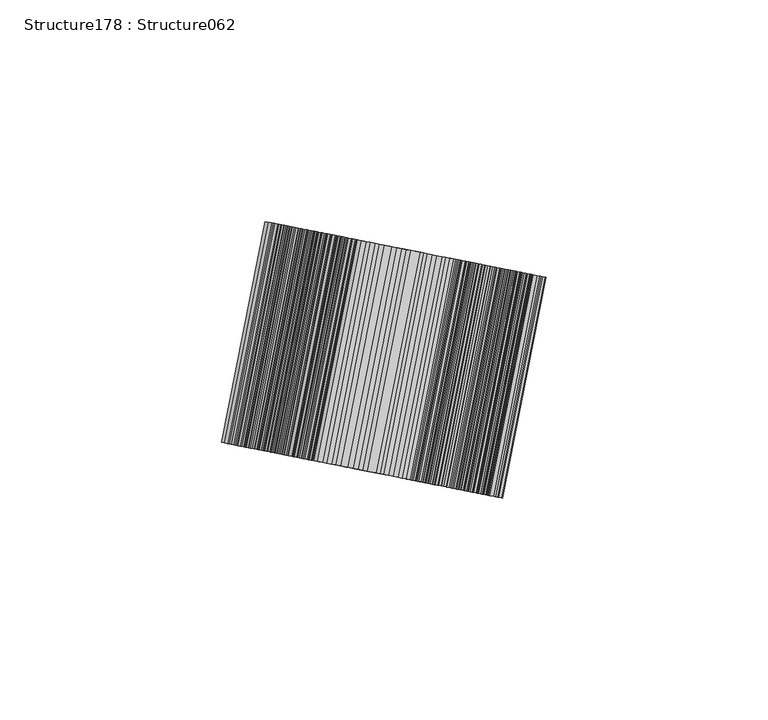
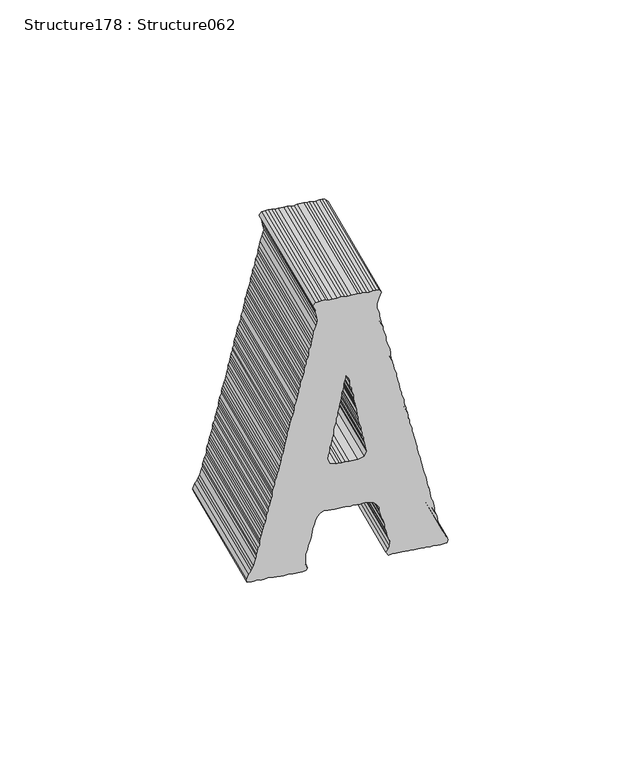
"""IFC4 building model written with IfcOpenShell, lengths in millimetres: proxy geometry, Structure178 : Structure062."""

from ifc_helpers import new_model, si_unit, frame, origin, place, context, project, spatial, polyline, outline, extrude, source, transform, mapped, element, save


def structure178_structure062_75744fdd(model_context):
    return source(origin(), model_context, "Body", "SweptSolid", [
        extrude(outline(polyline([(0.9094651, 0.0), (2.0811665, -0.5191353), (2.9906316, -0.6475848), (4.1562841, -0.7760343), (5.1991801, -1.1663642), (5.9748585, -1.299795), (7.1504738, -1.6851435), (8.1894559, -1.6851435), (9.3551084, -2.0758292), (10.2645735, -2.3377097), (11.4362748, -2.5946087), (12.3453841, -2.8564891), (13.3818755, -2.9849386), (14.1582655, -3.3752685), (15.4626861, -3.5040738), (16.3721513, -3.5040738), (17.5385154, -3.7659542), (19.491944, -4.4181645), (20.2718921, -4.6750635), (21.3101626, -4.9369439), (22.3470097, -4.9369439), (23.2561191, -5.1941987), (24.4278204, -5.5845287), (25.4700048, -5.9748585), (26.6363689, -5.9748585), (27.4124031, -6.3651884), (28.7175354, -6.6220874), (30.535754, -7.0127732), (31.5743802, -7.1462041), (32.7400327, -7.4031031), (33.6555467, -7.7934329), (35.4741211, -7.7934329), (36.5102567, -7.5315526), (37.5492387, -7.2746536), (38.3288311, -6.8843237), (39.3671015, -6.3651884), (40.4099976, -7.2746536), (40.5395145, -8.1837628), (40.5395145, -9.093228), (40.2826155, -10.2645735), (40.2826155, -11.3021323), (40.5395145, -12.4684964), (40.4099976, -13.2491562), (40.5395145, -14.1586213), (40.5395145, -16.2390762), (40.2826155, -17.2769908), (40.2826155, -18.3195311), (40.5395145, -19.4858951), (40.4099976, -20.6572406), (40.4099976, -22.3423842), (40.2826155, -23.5137297), (40.5395145, -24.422839), (40.5395145, -25.5941845), (40.4099976, -26.5032939), (40.2826155, -27.6746394), (39.2382962, -28.4506736), (38.3288311, -27.9315384), (37.4197218, -27.6746394), (36.6397736, -27.5412084), (35.4741211, -27.2843094), (33.5199809, -26.8939796), (32.6112274, -27.1508785), (31.4448633, -27.4127589), (29.3636968, -28.1934188), (27.545834, -28.4506736), (26.5089869, -28.712554), (25.3372855, -28.8410035), (24.2943895, -29.102884), (23.2561191, -29.6216633), (21.3101626, -29.7501128), (20.2718921, -30.012349), (19.491944, -30.5311284), (18.3202426, -30.5311284), (17.2816164, -30.9214584), (16.3721513, -31.1833388), (15.3356599, -31.1833388), (14.1582655, -31.4402377), (13.1253323, -31.8309234), (12.2158672, -32.2212534), (11.4362748, -32.3497029), (10.2645735, -32.4781524), (9.3551083, -32.8684823), (8.1894559, -32.8684823), (7.1504738, -33.259168), (6.2374505, -33.3876175), (5.0714422, -33.6494978), (3.2475306, -34.2967268), (2.0811665, -34.2967268), (1.1720572, -34.5586072), (0.1334309, -34.815862), (-1.0382704, -35.3396229), (-1.8178628, -35.4680724), (-2.8568449, -35.7249713), (-3.8990293, -35.8584022), (-5.0653934, -36.2487321), (-5.8471206, -36.5059869), (-7.0166871, -36.5059869), (-8.1826954, -36.8963168), (-8.9644226, -37.0297478), (-10.1364798, -37.4150963), (-11.1690572, -37.5485272), (-12.2115974, -37.6769766), (-12.9915456, -37.938857), (-14.03373, -38.3245613), (-15.3292552, -38.4579923), (-16.3678815, -38.7148912), (-18.1861001, -39.1052212), (-19.3581573, -39.3671016), (-20.2672666, -39.7528059), (-21.4371888, -40.0146862), (-22.2189161, -40.2765667), (-23.1223323, -40.5334657), (-24.1648726, -40.5334657), (-25.465735, -41.0572265), (-26.5025822, -41.3141255), (-27.4173846, -41.4429308), (-28.4560108, -41.4429308), (-29.235959, -41.7048112), (-30.5311284, -42.0951412), (-31.3110766, -42.2235906), (-32.3536168, -42.6139205), (-33.5214042, -42.6139205), (-34.4308693, -43.1330557), (-35.3399786, -43.3949362), (-36.37647, -43.3949362), (-37.5424783, -43.6568166), (-38.7202285, -44.0421651), (-39.6236447, -44.3040454), (-40.405372, -44.5659258), (-41.5752942, -44.6897497), (-42.6139205, -45.0850611), (-43.7856218, -45.3419601), (-44.8221132, -45.3419601), (-45.7372714, -45.4704096), (-46.6406876, -45.9941704), (-47.812389, -46.2510694), (-48.8510152, -46.5133056), (-49.7601245, -46.5133056), (-50.6731478, -46.9036355), (-52.8777823, -47.5508644), (-53.7929405, -47.9411943), (-54.5689747, -48.3318801), (-55.738897, -49.1125398), (-57.5532016, -49.7601246), (-58.4665807, -49.5028697), (-58.5957419, -48.1984491), (-58.4665807, -47.4224149), (-58.3331498, -46.2510694), (-58.5957419, -45.2135106), (-58.5957419, -44.0421651), (-58.3331498, -43.0042504), (-58.3331498, -42.0951412), (-58.4665807, -41.0572265), (-58.4665807, -40.1481172), (-58.5957419, -38.8433407), (-58.5957419, -37.938857), (-58.4665807, -36.8963168), (-58.3331498, -35.7249713), (-58.5957419, -34.815862), (-58.5957419, -31.8309234), (-58.3331498, -30.6595779), (-57.4297336, -30.1407985), (-56.6480063, -30.5311284), (-55.6115149, -30.7880274), (-53.3972734, -30.7880274), (-52.3586471, -30.7880274), (-51.4495378, -30.5311284), (-50.6731478, -30.1407985), (-49.3683714, -30.012349), (-48.4592621, -29.7501128), (-47.5497969, -29.3597829), (-46.6406876, -29.102884), (-45.6038405, -28.8410035), (-43.2661308, -28.5841045), (-41.5752942, -27.9315384), (-40.2762109, -27.6746394), (-38.9767716, -27.022429), (-38.1950444, -26.112964), (-37.4190102, -24.6847195), (-37.6759092, -23.6471606), (-37.6759092, -21.56635), (-37.5424783, -20.2669108), (-37.5424783, -17.5388712), (-37.6759092, -16.3675257), (-37.4190102, -15.4584164), (-37.5424783, -14.4205017), (-37.6759092, -13.3825872), (-37.5424783, -12.4684964), (-37.4190102, -11.1736828), (-37.6759092, -10.393023), (-38.0676623, -8.836329), (-38.8476105, -8.0503319), (-40.2762109, -7.0127732), (-41.4422191, -7.0127732), (-42.6139205, -6.7555183), (-44.561656, -6.2367389), (-45.3472973, -5.7129781), (-46.5133056, -5.4560792), (-47.2932538, -5.3276297), (-48.33188, -5.3276297), (-49.3683714, -4.803513), (-50.4126907, -4.6750635), (-51.4495378, -4.546614), (-52.3586471, -4.1562841), (-53.6595096, -3.7659542), (-55.3489229, -3.8944037), (-56.6480063, -4.2847336), (-57.2966585, -4.9369439), (-58.5957419, -4.1562841), (-58.4665807, -2.9849386), (-58.3331498, -1.9473797), (-58.3331498, 0.1334309), (-58.4665807, 1.1709896), (-58.4665807, 2.2089043), (-58.3331498, 3.1183694), (-58.4665807, 4.0274787), (-58.4665807, 5.3272737), (-58.3331498, 6.1079336), (-58.4665807, 7.4077285), (-58.3331498, 8.1887442), (-58.5957419, 9.2263031), (-58.3331498, 10.3976485), (-58.5957419, 11.5640127), (-58.4665807, 12.473122), (-58.3331498, 13.516018), (-58.3331498, 14.5535768), (-57.2966585, 14.9442625), (-56.3875492, 14.6823821), (-55.738897, 14.0347974), (-54.5689747, 13.7729169), (-53.7929405, 13.3825871), (-52.6151903, 12.8634519), (-50.6731478, 11.9543425), (-49.8875066, 11.6974435), (-48.5941162, 11.5640127), (-47.5497969, 11.3067579), (-46.6406876, 11.0448775), (-45.8646534, 10.6545475), (-44.561656, 10.526098), (-42.6139205, 10.2642176), (-41.4422191, 9.8788691), (-40.5384471, 9.4832021), (-39.6236447, 9.2263031), (-38.4576364, 9.0978536), (-37.4190102, 8.9644226), (-36.5059869, 8.8359731), (-35.6004358, 8.3171937), (-34.2956593, 8.1887442), (-33.3922431, 8.0553133), (-32.3536168, 7.926508), (-31.4405935, 7.536178), (-30.4019673, 7.1458482), (-29.235959, 6.8889492), (-27.5447666, 6.6270688), (-26.3752002, 6.2363831), (-25.203143, 6.1079336), (-24.4235506, 5.8510346), (-23.3849244, 5.4557232), (-22.4793732, 5.3272737), (-21.3037579, 4.9419253), (-20.2672666, 4.9419253), (-19.3581573, 4.6796891), (-18.319531, 4.4227901), (-17.1474738, 4.1609096), (-15.2018732, 3.6371488), (-14.1632469, 3.3802498), (-13.1207067, 3.3802498), (-12.2115974, 2.9895642), (-11.3024881, 2.5992342), (-10.0012698, 2.5992342), (-9.2270147, 2.0804548), (-8.1826954, 2.0804548), (-7.0166871, 1.9520053), (-5.9745027, 1.4328701), (-5.0653934, 1.4328701), (-4.1619771, 0.9140907), (-2.8568449, 0.7806597), (-1.9473797, 0.7806597), (-0.7817273, 0.2618804), (0.0, 0.0), (0.9094651, 0.0)]), holes=[polyline([(-20.9137838, -13.9017224), (-20.9137838, -16.8866609), (-20.7903157, -18.0576507), (-21.0472147, -19.2289961), (-20.7903157, -20.1384613), (-20.9137838, -21.0475706), (-20.2672666, -22.9945945), (-18.5817672, -23.6471606), (-17.2809048, -23.3852802), (-16.3678815, -23.123044), (-15.4623303, -22.866145), (-14.1632469, -22.9945945), (-13.2480888, -22.4758151), (-12.2115974, -22.3423842), (-11.3024881, -22.2139347), (-10.393023, -21.8285862), (-9.3508386, -21.6951553), (-8.3122123, -21.6951553), (-7.146204, -21.56635), (-6.3644768, -21.17602), (-5.3276296, -20.9141396), (-4.2854452, -20.9141396), (-3.117302, -20.3953603), (-1.9473797, -20.3953603), (-1.0382704, -20.0050304), (-0.2561874, -19.8762251), (1.0389821, -19.7477756), (2.0811665, -19.4858951), (3.1180136, -19.2289961), (4.0274787, -19.0955652), (5.0714422, -19.0955652), (6.1082894, -18.5767858), (7.0177545, -18.4483364), (8.1894559, -18.4483364), (9.2216774, -18.0576507), (10.1368356, -17.8007517), (11.0463007, -17.8007517), (10.1368356, -17.1485413), (9.0928721, -16.7582114), (8.056025, -16.6294061), (6.8900167, -16.6294061), (6.1082894, -16.1106267), (4.9365881, -15.9771958), (3.1180136, -15.4584164), (1.8189302, -15.3299669), (0.9094651, -15.2015174), (0.0, -14.9392812), (-1.0382704, -14.8108317), (-2.2078369, -14.4205017), (-4.2854452, -14.2920522), (-5.3276296, -14.0301719), (-6.3644768, -13.9017224), (-8.1826954, -13.5113925), (-9.2270147, -12.9922572), (-10.2638619, -12.9922572), (-11.1690572, -12.7303768), (-12.3446725, -12.6019273), (-13.1207067, -12.2115974), (-14.286715, -12.2115974), (-15.4623303, -11.8212676), (-17.2809048, -11.5590313), (-18.5817672, -11.3021323), (-20.1377496, -12.083148), (-20.9137838, -13.9017224)])]), frame((-2218.3415747, 234908.7270034, 444.9951864), z_axis=(0.19466222296394123, 0.9808703374813295, 0.0), x_axis=(0.0, 0.0, 1.0)), (0.0, 0.0, 1.0), 50.8),
    ])


if __name__ == "__main__":
    model = new_model("IFC4")
    model_context = context("Model", 3, world=origin())
    ifc_project = project(units=[si_unit("LENGTHUNIT", "METRE", prefix="MILLI")], contexts=[model_context])
    site = spatial("IfcSite", under=ifc_project)
    building = spatial("IfcBuilding", under=site)
    placement = place(None, origin())
    structure178_structure062_shape = structure178_structure062_75744fdd(model_context)
    element("IfcBuildingElementProxy", 1, Name="Structure178 : Structure062", ObjectType="Structure178 : Structure062", at=placement, inside=building, context=model_context, shape_type="MappedRepresentation", body=[
        mapped(structure178_structure062_shape, transform((0.0, 0.0, 0.0), x_axis=(1.0, 0.0, 0.0), y_axis=(0.0, 1.0, 0.0), z_axis=(0.0, 0.0, 1.0))),
    ])
    save(model, "model.ifc")

# Revit data of these elements
# Type "Structure178 : Structure062"
#   NameOverride = "Structure062"
# Element 1 (IfcBuildingElementProxy, "Structure178 : Structure062")
#   Materials on its faces: "BRUSHED ALUMINUM LETTERING"
# Materials
#   "BRUSHED ALUMINUM LETTERING": class "Unassigned", colour RGB 169 181 186, transparency 0, Cost = 0
